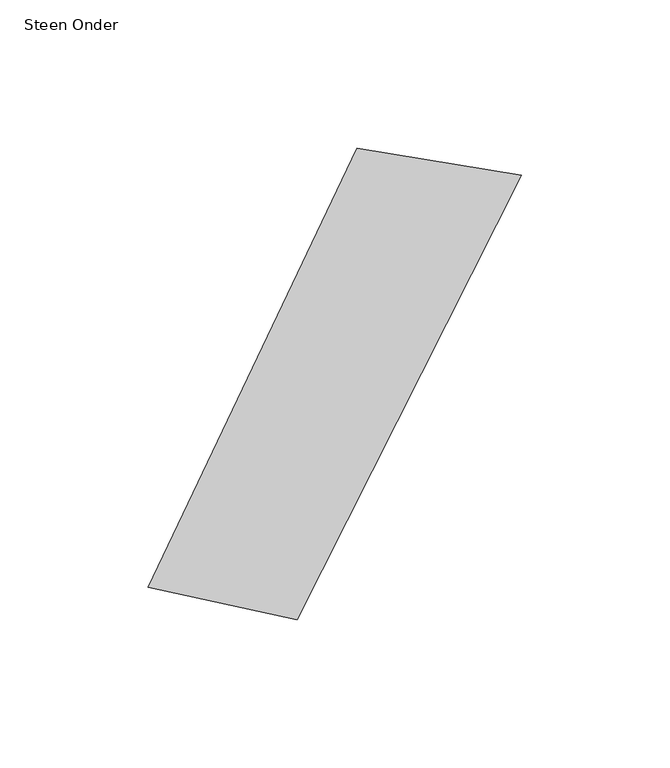
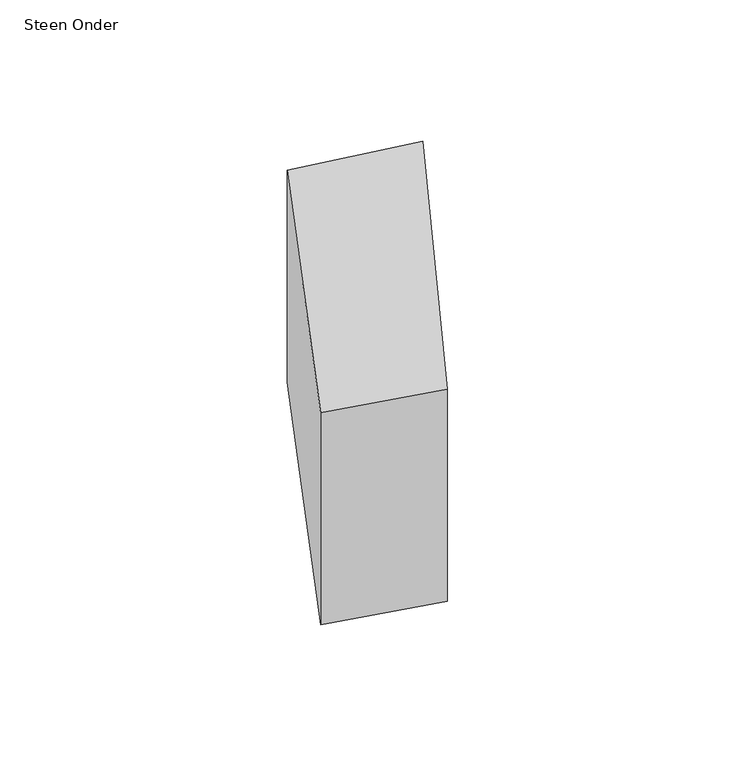
"""IFC4 building model written with IfcOpenShell, lengths in millimetres: proxy geometry, 00_GMA_steen_versie_4 : Steen Onder."""

from ifc_helpers import new_model, si_unit, origin, origin_with_axes, place, context, project, spatial, polyline, outline, extrude, source, transform, mapped, element, save


def steen_onder_7f6d7dc1(model_context):
    return source(origin(), model_context, "Body", "SweptSolid", [
        extrude(outline(polyline([(137.3024219, 142.1509937), (61.7503655, -7.467366), (11.6022569, 3.3124147), (81.9382935, 151.1923817), (137.3024219, 142.1509937)])), origin_with_axes(), (0.0, 0.0, 1.0), 100.0),
    ])


if __name__ == "__main__":
    model = new_model("IFC4")
    model_context = context("Model", 3, world=origin())
    ifc_project = project(units=[si_unit("LENGTHUNIT", "METRE", prefix="MILLI")], contexts=[model_context])
    site = spatial("IfcSite", under=ifc_project)
    building = spatial("IfcBuilding", under=site)
    placement = place(None, origin())
    steen_onder_shape = steen_onder_7f6d7dc1(model_context)
    element("IfcBuildingElementProxy", 1, Name="00_GMA_steen_versie_4 : Steen Onder", ObjectType="00_GMA_steen_versie_4 : Steen Onder", at=placement, inside=building, context=model_context, shape_type="MappedRepresentation", body=[
        mapped(steen_onder_shape, transform((0.0, 0.0, 0.0), x_axis=(1.0, 0.0, 0.0), y_axis=(0.0, 1.0, 0.0), z_axis=(0.0, 0.0, 1.0))),
    ])
    save(model, "model.ifc")

# Revit data of these elements
# Type "00_GMA_steen_versie_4 : Steen Onder"
#   StootVoegHalfBoven [instance default] = 5 mm
#   StootVoegHalf [instance default] = 5 mm
#   StootVoegBreedteOnder = 10 mm
#   StootVoegBreedteBoven = 10 mm
#   Steendikte = 100 mm
#   LintVoegOnderHalf = 0 mm
#   LintVoegOnder = 0 mm
#   LintVoegBovenHalf = 5 mm
#   LintVoegBoven = 10 mm
#   materiaal = none
#   MateriaalVoeg = none
#   Default Elevation = 0
